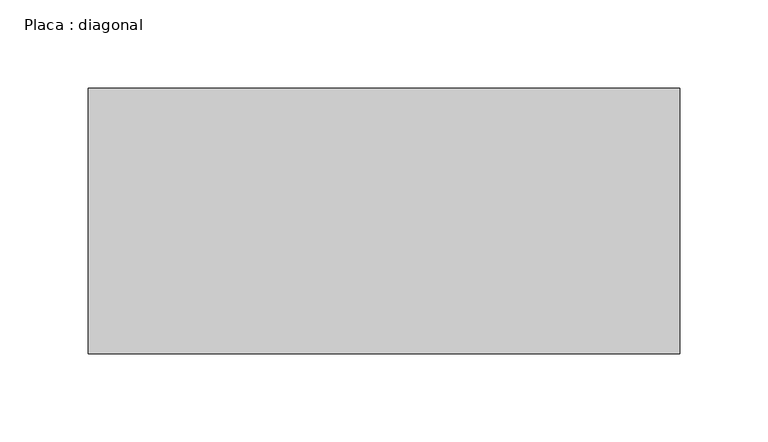
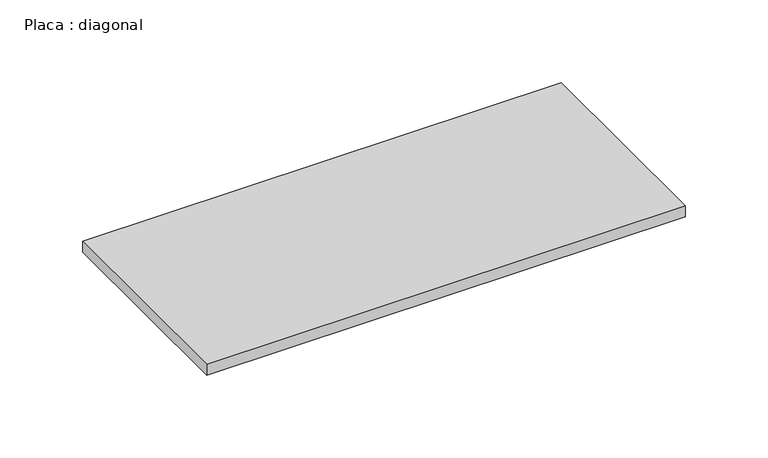
"""IFC4 building model written with IfcOpenShell, lengths in millimetres: beam geometry, Placa : diagonal."""

from ifc_helpers import new_model, si_unit, frame, origin, place, context, project, spatial, polyline, outline, extrude, source, transform, mapped, element, save


def placa_diagonal_aaf0c3b6(model_context):
    return source(origin(), model_context, "Body", "SweptSolid", [
        extrude(outline(polyline([(167.4240163, 75.0), (167.4240163, -75.0), (-167.067539, -75.0), (-167.067539, 75.0), (167.4240163, 75.0)])), frame((0.0, 0.0, -4.0), z_axis=(0.0, 0.0, 1.0), x_axis=(1.0, 0.0, 0.0)), (0.0, 0.0, 1.0), 8.0),
    ])


if __name__ == "__main__":
    model = new_model("IFC4")
    model_context = context("Model", 3, world=origin())
    ifc_project = project(units=[si_unit("LENGTHUNIT", "METRE", prefix="MILLI")], contexts=[model_context])
    site = spatial("IfcSite", under=ifc_project)
    building = spatial("IfcBuilding", under=site)
    placement = place(None, origin())
    placa_diagonal_shape = placa_diagonal_aaf0c3b6(model_context)
    element("IfcBeam", 1, ObjectType="Placa : diagonal", at=placement, inside=building, context=model_context, shape_type="MappedRepresentation", body=[
        mapped(placa_diagonal_shape, transform((0.0, 0.0, 0.0), x_axis=(1.0, 0.0, 0.0), y_axis=(0.0, 1.0, 0.0), z_axis=(0.0, 0.0, 1.0))),
    ])
    save(model, "model.ifc")

# Revit data of these elements
# Type "Placa : diagonal"
#   W = 0
#   Length [instance default] = 1.50 m
#   b = 0.15 m
#   d = 0.008 m
#   A = 0 m²
#   Structural Material [instance default] = Aço, 45-345
# Element 1 (IfcBeam, "Placa : diagonal")
#   Materials on its faces: "Aço, 45-345"
# Materials
#   "Aço, 45-345": class "Metal", colour RGB 247 247 247, transparency 0, Description = "Aço 345 MPa", Cost = 0
